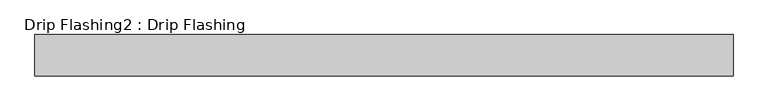
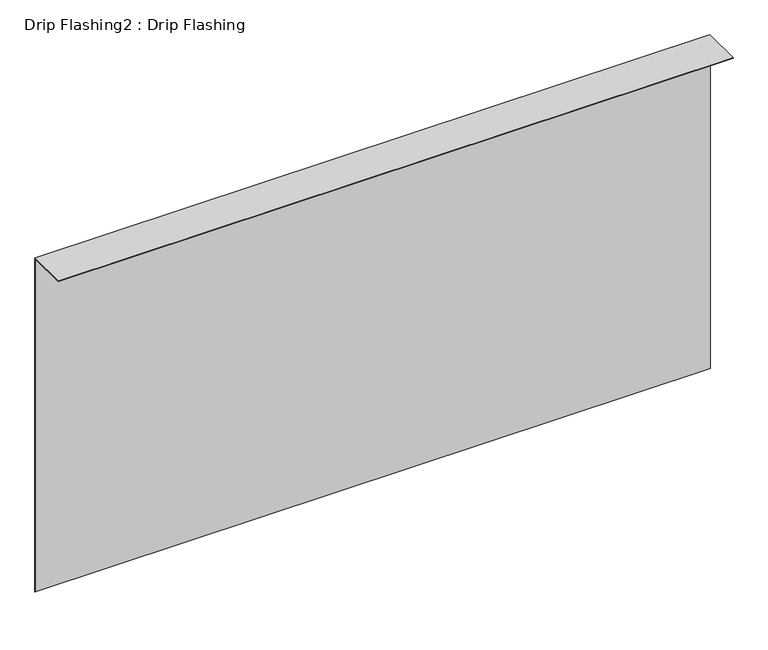
"""IFC4 building model written with IfcOpenShell, lengths in millimetres: proxy geometry, Drip Flashing2 : Drip Flashing."""

from ifc_helpers import new_model, si_unit, frame, origin, place, context, project, spatial, polyline, outline, extrude, source, transform, mapped, element, save


def drip_flashing2_drip_flashing_0b339f89(model_context):
    return source(origin(), model_context, "Body", "SweptSolid", [
        extrude(outline(polyline([(9742.7912647, 37600.3015275), (9625.4543522, 37600.3015275), (9625.4543522, 37601.8015275), (9744.2912647, 37601.8015275), (9744.2912647, 36556.696), (9742.7912647, 36556.696), (9742.7912647, 37600.3015275)])), frame((-9232.0719278, 0.0, 0.0), z_axis=(1.0, 0.0, 0.0), x_axis=(0.0, 1.0, 0.0)), (0.0, 0.0, 1.0), 1999.85),
    ])


if __name__ == "__main__":
    model = new_model("IFC4")
    model_context = context("Model", 3, world=origin())
    ifc_project = project(units=[si_unit("LENGTHUNIT", "METRE", prefix="MILLI")], contexts=[model_context])
    site = spatial("IfcSite", under=ifc_project)
    building = spatial("IfcBuilding", under=site)
    placement = place(None, origin())
    drip_flashing2_drip_flashing_shape = drip_flashing2_drip_flashing_0b339f89(model_context)
    element("IfcBuildingElementProxy", 1, Name="Drip Flashing2 : Drip Flashing", ObjectType="Drip Flashing2 : Drip Flashing", at=placement, inside=building, context=model_context, shape_type="MappedRepresentation", body=[
        mapped(drip_flashing2_drip_flashing_shape, transform((0.0, 0.0, 0.0), x_axis=(1.0, 0.0, 0.0), y_axis=(0.0, 1.0, 0.0), z_axis=(0.0, 0.0, 1.0))),
    ])
    save(model, "model.ifc")

# Revit data of these elements
# Project information
#   Issued Date 1 = "0/00/2018 - City of Newport Beach"
#   IfcSite GUID = "3hCLsSIbaHwOLX093rt3ko"
#   IfcBuilding GUID = "3hCN2YIbaHwOLX093rt3ko"
#   IfcProject GUID = "7043067b_ee86_4e71_a94"
#   NameOverride = "Default Site"
#   Project Issue Date = "Issue Date"
#   Project Status = "Project Status"
#   Client Name = "xxx"
#   Project Address = "xxx"
#   Project Name = "STAUDENMEIER RESIDENCE"
# Type "Drip Flashing2 : Drip Flashing"
#   NameOverride = "Drip Flashing"
# Element 1 (IfcBuildingElementProxy, "Drip Flashing2 : Drip Flashing")
#   Materials on its faces: "(2) LAYERS OF ICE & WATER SHIELD (BITUTHANE) UNDER STUCCO"
# Materials
#   "(2) LAYERS OF ICE & WATER SHIELD (BITUTHANE) UNDER STUCCO": class "Unassigned", colour RGB 186 255 159, transparency 0, Cost = 0
